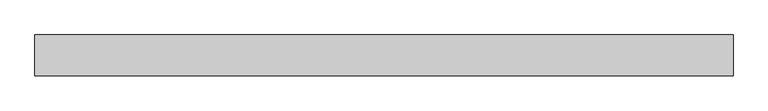
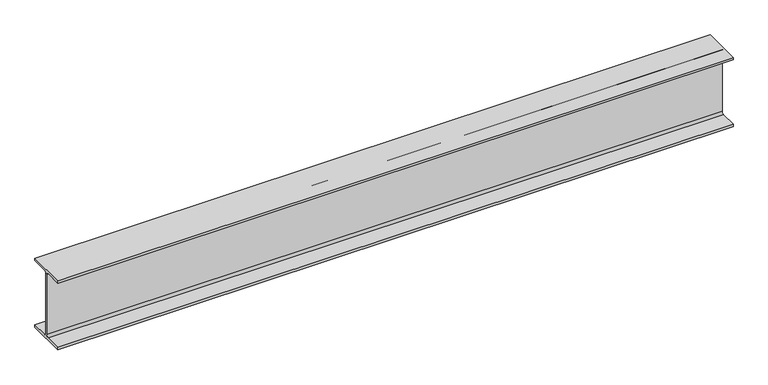
"""IFC4 building model written with IfcOpenShell, lengths in millimetres: beam geometry, Old_Steel Beam_H-KSD3502 : H_SB_ASB_H-250×125x6x9."""

from ifc_helpers import new_model, si_unit, point, frame, frame_2d, origin, place, context, project, spatial, polyline, circle_curve, trimmed, segment, composite_curve, outline, extrude, source, transform, mapped, element, save


def beam_8c7e44f5(model_context):
    return source(origin(), model_context, "Body", "SweptSolid", [
        extrude(outline(composite_curve([segment(polyline([(82.5, -141.5), (82.5, -151.7), (-82.5, -151.7), (-82.5, -141.5), (-11.9, -141.5)]), True, "CONTINUOUS"), segment(trimmed(circle_curve(frame_2d((-11.9, -132.6)), 8.9), [point((-11.9, -141.5))], [point((-3.0, -132.6))], True, "CARTESIAN"), True, "CONTINUOUS"), segment(polyline([(-3.0, -132.6), (-3.0, 132.6)]), True, "CONTINUOUS"), segment(trimmed(circle_curve(frame_2d((-11.9, 132.6)), 8.9), [point((-3.0, 132.6))], [point((-11.9, 141.5))], True, "CARTESIAN"), True, "CONTINUOUS"), segment(polyline([(-11.9, 141.5), (-82.5, 141.5), (-82.5, 151.7), (82.5, 151.7), (82.5, 141.5), (11.9, 141.5)]), True, "CONTINUOUS"), segment(trimmed(circle_curve(frame_2d((11.9, 132.6)), 8.9), [point((11.9, 141.5))], [point((3.0, 132.6))], True, "CARTESIAN"), True, "CONTINUOUS"), segment(polyline([(3.0, 132.6), (3.0, -132.6)]), True, "CONTINUOUS"), segment(trimmed(circle_curve(frame_2d((11.9, -132.6)), 8.9), [point((3.0, -132.6))], [point((11.9, -141.5))], True, "CARTESIAN"), True, "CONTINUOUS"), segment(polyline([(11.9, -141.5), (82.5, -141.5)]), True, "CONTINUOUS")], self_intersect=False)), frame((-1404.8000503, 0.0, 0.0), z_axis=(1.0, 0.0, 0.0), x_axis=(0.0, 1.0, 0.0)), (0.0, 0.0, 1.0), 2809.5192866),
    ])


if __name__ == "__main__":
    model = new_model("IFC4")
    model_context = context("Model", 3, world=origin())
    ifc_project = project(units=[si_unit("LENGTHUNIT", "METRE", prefix="MILLI")], contexts=[model_context])
    site = spatial("IfcSite", under=ifc_project)
    building = spatial("IfcBuilding", under=site)
    placement = place(None, origin())
    beam_shape = beam_8c7e44f5(model_context)
    element("IfcBeam", 1, ObjectType="Old_Steel Beam_H-KSD3502 : H_SB_ASB_H-250×125x6x9", at=placement, inside=building, context=model_context, shape_type="MappedRepresentation", body=[
        mapped(beam_shape, transform((0.0, 0.0, 0.0), x_axis=(1.0, 0.0, 0.0), y_axis=(0.0, 1.0, 0.0), z_axis=(0.0, 0.0, 1.0))),
    ])
    save(model, "model.ifc")

# Revit data of these elements
# Type "Old_Steel Beam_H-KSD3502 : H_SB_ASB_H-250×125x6x9"
#   Width = 12.5 cm
#   Web Thickness = 0.6 cm
#   Web Fillet = 1.2 cm
#   Warping Constant = 42539.8 cm⁶
#   Torsional Moment of Inertia = 7.8102 cm⁴
#   Torsional Modulus = 1.0 cm³
#   Section Area = 37.66 cm²
#   Plastic Modulus weak axis = 73.1 cm³
#   Plastic Modulus strong axis = 366.0 cm³
#   Perimeter = 0.97 m²/m
#   Nominal Weight = 29.60 kgf/m
#   Moment of Inertia weak axis = 294.00 cm⁴
#   Moment of Inertia strong axis = 4050.00 cm⁴
#   Height = 25.0 cm
#   Flange Thickness = 0.9 cm
#   Elastic Modulus weak axis = 47.0 cm³
#   Elastic Modulus strong axis = 324.0 cm³
#   Centroid Vertical = 12.5 cm
#   Centroid Horizontal = 6.25 cm
#   Length [instance default] = 1.5240 m
#   Structural Material [instance default] = Steel, 45-345
#   Assembly Code = ""
# Element 1 (IfcBeam, "Old_Steel Beam_H-KSD3502 : H_SB_ASB_H-250×125x6x9")
#   Structural Material = none
# Materials
#   "Steel, 45-345": class "Metal", colour RGB 189 187 185, transparency 0, Description = "Steel 345 MPa", Cost = 0
